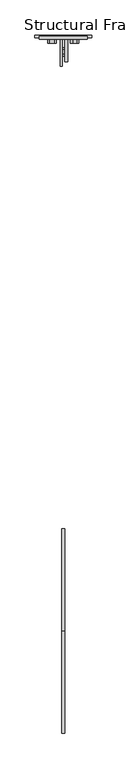
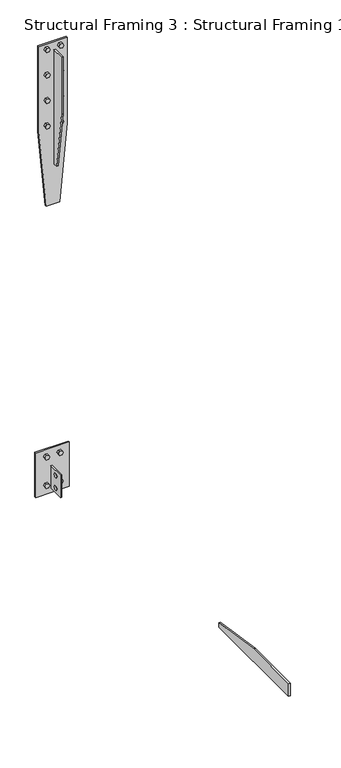
"""IFC4 building model written with IfcOpenShell, lengths in millimetres: beam geometry, Structural Framing 3 : Structural Framing 1."""

from ifc_helpers import new_model, si_unit, frame, origin, place, context, project, spatial, polyline, outline, extrude, source, transform, mapped, element, save


def structural_framing_3_structural_framing_1_6b3e3b3d(model_context):
    return source(origin(), model_context, "Body", "SweptSolid", [
        extrude(outline(polyline([(-74.0021465, 3361.7022161), (-93.0521465, 3361.7022161), (-102.5771465, 3378.2), (-93.0521465, 3394.6977839), (-74.0021465, 3394.6977839), (-64.4771465, 3378.2), (-74.0021465, 3361.7022161)])), frame((-1843.2423771, 0.0, 0.0), z_axis=(1.0, 0.0, 0.0), x_axis=(0.0, 1.0, 0.0)), (0.0, 0.0, 1.0), 19.05),
        extrude(outline(polyline([(-74.0021465, 3295.1297839), (-64.4771465, 3278.632), (-74.0021465, 3262.1342161), (-93.0521465, 3262.1342161), (-102.5771465, 3278.632), (-93.0521465, 3295.1297839), (-74.0021465, 3295.1297839)])), frame((-1843.2423771, 0.0, 0.0), z_axis=(1.0, 0.0, 0.0), x_axis=(0.0, 1.0, 0.0)), (0.0, 0.0, 1.0), 19.05),
        extrude(outline(polyline([(-1833.7173771, -147.0271465), (-1843.2423771, -147.0271465), (-1843.2423771, -20.0271465), (-1833.7173771, -20.0271465), (-1833.7173771, -147.0271465)])), frame((0.0, 0.0, 3239.516), z_axis=(0.0, 0.0, 1.0), x_axis=(1.0, 0.0, 0.0)), (0.0, 0.0, 1.0), 177.8),
        extrude(outline(polyline([(3295.1297839, -1769.3918771), (3295.1297839, -1788.4418771), (3278.632, -1797.9668771), (3262.1342161, -1788.4418771), (3262.1342161, -1769.3918771), (3278.632, -1759.8668771), (3295.1297839, -1769.3918771)])), frame((0.0, -39.0771465, 0.0), z_axis=(0.0, 1.0, 0.0), x_axis=(0.0, 0.0, 1.0)), (0.0, 0.0, 1.0), 19.05),
        extrude(outline(polyline([(3523.7297839, -1769.3918771), (3523.7297839, -1788.4418771), (3507.232, -1797.9668771), (3490.7342161, -1788.4418771), (3490.7342161, -1769.3918771), (3507.232, -1759.8668771), (3523.7297839, -1769.3918771)])), frame((0.0, -39.0771465, 0.0), z_axis=(0.0, 1.0, 0.0), x_axis=(0.0, 0.0, 1.0)), (0.0, 0.0, 1.0), 19.05),
        extrude(outline(polyline([(3295.1297839, -1890.0418771), (3278.632, -1899.5668771), (3262.1342161, -1890.0418771), (3262.1342161, -1870.9918771), (3278.632, -1861.4668771), (3295.1297839, -1870.9918771), (3295.1297839, -1890.0418771)])), frame((0.0, -39.0771465, 0.0), z_axis=(0.0, 1.0, 0.0), x_axis=(0.0, 0.0, 1.0)), (0.0, 0.0, 1.0), 19.05),
        extrude(outline(polyline([(3523.7297839, -1890.0418771), (3507.232, -1899.5668771), (3490.7342161, -1890.0418771), (3490.7342161, -1870.9918771), (3507.232, -1861.4668771), (3523.7297839, -1870.9918771), (3523.7297839, -1890.0418771)])), frame((0.0, -39.0771465, 0.0), z_axis=(0.0, 1.0, 0.0), x_axis=(0.0, 0.0, 1.0)), (0.0, 0.0, 1.0), 19.05),
        extrude(outline(polyline([(-1956.7168771, -7.3271465), (-1702.7168771, -7.3271465), (-1702.7168771, -20.0271465), (-1956.7168771, -20.0271465), (-1956.7168771, -7.3271465)])), frame((0.0, 0.0, 3202.432), z_axis=(0.0, 0.0, 1.0), x_axis=(1.0, 0.0, 0.0)), (0.0, 0.0, 1.0), 355.6),
        extrude(outline(polyline([(6175.9977839, -1788.4418771), (6159.5, -1797.9668771), (6143.0022161, -1788.4418771), (6143.0022161, -1769.3918771), (6159.5, -1759.8668771), (6175.9977839, -1769.3918771), (6175.9977839, -1788.4418771)])), frame((0.0, -45.4271465, 0.0), z_axis=(0.0, 1.0, 0.0), x_axis=(0.0, 0.0, 1.0)), (0.0, 0.0, 1.0), 19.05),
        extrude(outline(polyline([(6175.9977839, -1890.0418771), (6159.5, -1899.5668771), (6143.0022161, -1890.0418771), (6143.0022161, -1870.9918771), (6159.5, -1861.4668771), (6175.9977839, -1870.9918771), (6175.9977839, -1890.0418771)])), frame((0.0, -45.4271465, 0.0), z_axis=(0.0, 1.0, 0.0), x_axis=(0.0, 0.0, 1.0)), (0.0, 0.0, 1.0), 19.05),
        extrude(outline(polyline([(6379.1977839, -1788.4418771), (6362.7, -1797.9668771), (6346.2022161, -1788.4418771), (6346.2022161, -1769.3918771), (6362.7, -1759.8668771), (6379.1977839, -1769.3918771), (6379.1977839, -1788.4418771)])), frame((0.0, -45.4271465, 0.0), z_axis=(0.0, 1.0, 0.0), x_axis=(0.0, 0.0, 1.0)), (0.0, 0.0, 1.0), 19.05),
        extrude(outline(polyline([(6379.1977839, -1890.0418771), (6362.7, -1899.5668771), (6346.2022161, -1890.0418771), (6346.2022161, -1870.9918771), (6362.7, -1861.4668771), (6379.1977839, -1870.9918771), (6379.1977839, -1890.0418771)])), frame((0.0, -45.4271465, 0.0), z_axis=(0.0, 1.0, 0.0), x_axis=(0.0, 0.0, 1.0)), (0.0, 0.0, 1.0), 19.05),
        extrude(outline(polyline([(6582.3977839, -1788.4418771), (6565.9, -1797.9668771), (6549.4022161, -1788.4418771), (6549.4022161, -1769.3918771), (6565.9, -1759.8668771), (6582.3977839, -1769.3918771), (6582.3977839, -1788.4418771)])), frame((0.0, -45.4271465, 0.0), z_axis=(0.0, 1.0, 0.0), x_axis=(0.0, 0.0, 1.0)), (0.0, 0.0, 1.0), 19.05),
        extrude(outline(polyline([(6582.3977839, -1890.0418771), (6565.9, -1899.5668771), (6549.4022161, -1890.0418771), (6549.4022161, -1870.9918771), (6565.9, -1861.4668771), (6582.3977839, -1870.9918771), (6582.3977839, -1890.0418771)])), frame((0.0, -45.4271465, 0.0), z_axis=(0.0, 1.0, 0.0), x_axis=(0.0, 0.0, 1.0)), (0.0, 0.0, 1.0), 19.05),
        extrude(outline(polyline([(6785.5977839, -1788.4418771), (6769.1, -1797.9668771), (6752.6022161, -1788.4418771), (6752.6022161, -1769.3918771), (6769.1, -1759.8668771), (6785.5977839, -1769.3918771), (6785.5977839, -1788.4418771)])), frame((0.0, -45.4271465, 0.0), z_axis=(0.0, 1.0, 0.0), x_axis=(0.0, 0.0, 1.0)), (0.0, 0.0, 1.0), 19.05),
        extrude(outline(polyline([(6785.5977839, -1890.0418771), (6769.1, -1899.5668771), (6752.6022161, -1890.0418771), (6752.6022161, -1870.9918771), (6769.1, -1861.4668771), (6785.5977839, -1870.9918771), (6785.5977839, -1890.0418771)])), frame((0.0, -45.4271465, 0.0), z_axis=(0.0, 1.0, 0.0), x_axis=(0.0, 0.0, 1.0)), (0.0, 0.0, 1.0), 19.05),
        extrude(outline(polyline([(-3128.0411296, 3556.0), (-2670.8411296, 3556.0), (-2213.6411296, 3488.6697466), (-2213.6411296, 3454.4), (-3128.0411296, 3454.4), (-3128.0411296, 3556.0)])), frame((-1836.0668771, 0.0, 0.0), z_axis=(1.0, 0.0, 0.0), x_axis=(0.0, 1.0, 0.0)), (0.0, 0.0, 1.0), 12.7),
        extrude(outline(polyline([(-127.9771465, 6743.7), (-26.3771465, 6743.7), (-26.3771465, 5829.3), (-60.6468931, 5829.3), (-127.9771465, 6286.5), (-127.9771465, 6743.7)])), frame((-1823.3668771, 0.0, 0.0), z_axis=(1.0, 0.0, 0.0), x_axis=(0.0, 1.0, 0.0)), (0.0, 0.0, 1.0), 12.7),
        extrude(outline(polyline([(6121.4, -1721.7668771), (6807.2, -1721.7668771), (6807.2, -1937.6668771), (6121.4, -1937.6668771), (5511.8, -1880.5168771), (5511.8, -1778.9168771), (6121.4, -1721.7668771)])), frame((0.0, -26.3771465, 0.0), z_axis=(0.0, 1.0, 0.0), x_axis=(0.0, 0.0, 1.0)), (0.0, 0.0, 1.0), 12.7),
    ])


if __name__ == "__main__":
    model = new_model("IFC4")
    model_context = context("Model", 3, world=origin())
    ifc_project = project(units=[si_unit("LENGTHUNIT", "METRE", prefix="MILLI")], contexts=[model_context])
    site = spatial("IfcSite", under=ifc_project)
    building = spatial("IfcBuilding", under=site)
    placement = place(None, origin())
    structural_framing_3_structural_framing_1_shape = structural_framing_3_structural_framing_1_6b3e3b3d(model_context)
    element("IfcBeam", 1, ObjectType="Structural Framing 3 : Structural Framing 1", at=placement, inside=building, context=model_context, shape_type="MappedRepresentation", body=[
        mapped(structural_framing_3_structural_framing_1_shape, transform((0.0, 0.0, 0.0), x_axis=(1.0, 0.0, 0.0), y_axis=(0.0, 1.0, 0.0), z_axis=(0.0, 0.0, 1.0))),
    ])
    save(model, "model.ifc")

# Revit data of these elements
# Element 1 (IfcBeam, "Structural Framing 3 : Structural Framing 1")
#   Materials on its faces: "Galvanized Steel"
# Materials
#   "Galvanized Steel": class "Generic", colour RGB 232 232 232, transparency 0, Description = "Acoustic Ceiling Tile 24 x 24", Cost = 0
